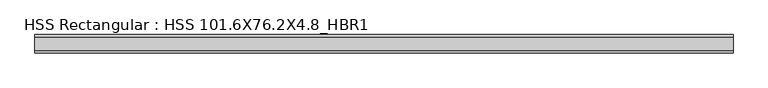
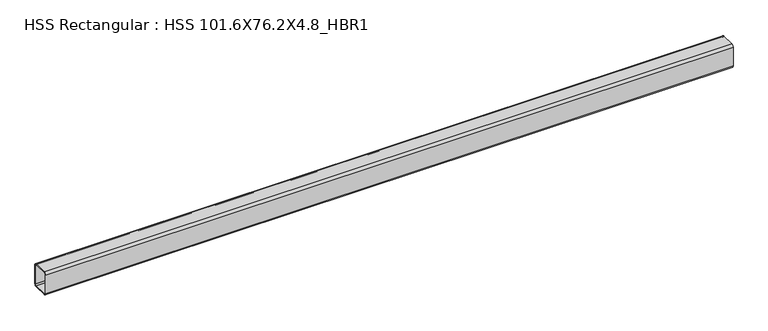
"""IFC4 building model written with IfcOpenShell, lengths in millimetres: beam geometry, HSS Rectangular : HSS 101.6X76.2X4.8_HBR1."""

from ifc_helpers import new_model, si_unit, point, frame, frame_2d, origin, place, context, project, spatial, polyline, circle_curve, trimmed, segment, composite_curve, outline, extrude, source, transform, mapped, element, save


def hss_rectangular_hss_101_6x76_2x4_8_hbr1_dbf90deb(model_context):
    return source(origin(), model_context, "Body", "SweptSolid", [
        extrude(outline(composite_curve([segment(polyline([(38.1, 41.275), (38.1, -41.275)]), True, "CONTINUOUS"), segment(trimmed(circle_curve(frame_2d((28.575, -41.275)), 9.525), [point((38.1, -41.275))], [point((28.575, -50.8))], False, "CARTESIAN"), True, "CONTINUOUS"), segment(polyline([(28.575, -50.8), (-28.575, -50.8)]), True, "CONTINUOUS"), segment(trimmed(circle_curve(frame_2d((-28.575, -41.275)), 9.525), [point((-28.575, -50.8))], [point((-38.1, -41.275))], False, "CARTESIAN"), True, "CONTINUOUS"), segment(polyline([(-38.1, -41.275), (-38.1, 41.275)]), True, "CONTINUOUS"), segment(trimmed(circle_curve(frame_2d((-28.575, 41.275)), 9.525), [point((-38.1, 41.275))], [point((-28.575, 50.8))], False, "CARTESIAN"), True, "CONTINUOUS"), segment(polyline([(-28.575, 50.8), (28.575, 50.8)]), True, "CONTINUOUS"), segment(trimmed(circle_curve(frame_2d((28.575, 41.275)), 9.525), [point((28.575, 50.8))], [point((38.1, 41.275))], False, "CARTESIAN"), True, "CONTINUOUS")], self_intersect=False), holes=[composite_curve([segment(trimmed(circle_curve(frame_2d((-28.575, 41.275)), 4.7625), [point((-28.575, 46.0375))], [point((-33.3375, 41.275))], True, "CARTESIAN"), True, "CONTINUOUS"), segment(polyline([(-33.3375, 41.275), (-33.3375, -41.275)]), True, "CONTINUOUS"), segment(trimmed(circle_curve(frame_2d((-28.575, -41.275)), 4.7625), [point((-33.3375, -41.275))], [point((-28.575, -46.0375))], True, "CARTESIAN"), True, "CONTINUOUS"), segment(polyline([(-28.575, -46.0375), (28.575, -46.0375)]), True, "CONTINUOUS"), segment(trimmed(circle_curve(frame_2d((28.575, -41.275)), 4.7625), [point((28.575, -46.0375))], [point((33.3375, -41.275))], True, "CARTESIAN"), True, "CONTINUOUS"), segment(polyline([(33.3375, -41.275), (33.3375, 41.275)]), True, "CONTINUOUS"), segment(trimmed(circle_curve(frame_2d((28.575, 41.275)), 4.7625), [point((33.3375, 41.275))], [point((28.575, 46.0375))], True, "CARTESIAN"), True, "CONTINUOUS"), segment(polyline([(28.575, 46.0375), (-28.575, 46.0375)]), True, "CONTINUOUS")], self_intersect=False)]), frame((-1376.6301953, 0.0, 0.0), z_axis=(1.0, 0.0, 0.0), x_axis=(0.0, 1.0, 0.0)), (0.0, 0.0, 1.0), 2906.597179),
    ])


if __name__ == "__main__":
    model = new_model("IFC4")
    model_context = context("Model", 3, world=origin())
    ifc_project = project(units=[si_unit("LENGTHUNIT", "METRE", prefix="MILLI")], contexts=[model_context])
    site = spatial("IfcSite", under=ifc_project)
    building = spatial("IfcBuilding", under=site)
    placement = place(None, origin())
    hss_rectangular_hss_101_6x76_2x4_8_hbr1_shape = hss_rectangular_hss_101_6x76_2x4_8_hbr1_dbf90deb(model_context)
    element("IfcBeam", 1, ObjectType="HSS Rectangular : HSS 101.6X76.2X4.8_HBR1", at=placement, inside=building, context=model_context, shape_type="MappedRepresentation", body=[
        mapped(hss_rectangular_hss_101_6x76_2x4_8_hbr1_shape, transform((0.0, 0.0, 0.0), x_axis=(1.0, 0.0, 0.0), y_axis=(0.0, 1.0, 0.0), z_axis=(0.0, 0.0, 1.0))),
    ])
    save(model, "model.ifc")

# Revit data of these elements
# Type "HSS Rectangular : HSS 101.6X76.2X4.8_HBR1"
#   Section Name Key = "HSS 4X3X3/16"
#   Assembly Code = "B10"
#   Width = 7.62 cm
#   Wall Nominal Thickness = 0.4763 cm
#   Wall Design Thickness = 0.442 cm
#   Torsional Moment of Inertia = 260.561 cm⁴
#   Torsional Modulus = 61.2876 cm³
#   Section Area = 14.4516 cm²
#   Plastic Modulus weak axis = 40.3122 cm³
#   Plastic Modulus strong axis = 49.1612 cm³
#   Perimeter = 0.881482 m²/m
#   Outer Fillet = 0.9525 cm
#   Nominal Weight = 12.1285 kgf/m
#   Moment of Inertia weak axis = 131.529 cm⁴
#   Moment of Inertia strong axis = 205.202 cm⁴
#   Inner Fillet = 0.4763 cm
#   Height = 10.16 cm
#   Elastic Modulus weak axis = 34.4128 cm³
#   Elastic Modulus strong axis = 40.476 cm³
#   Centroid Vertical = 5.08 cm
#   Centroid Horizontal = 3.81 cm
#   Length [instance default] = 1524 mm
#   Structural Material [instance default] = Steel ASTM A500, Grade B, Rectangular and Square
#   Principal Axes Angle = 0
# Element 1 (IfcBeam, "HSS Rectangular : HSS 101.6X76.2X4.8_HBR1")
#   Structural Material = Steel ASTM A992
#   Materials on its faces: "Steel ASTM A992"
# Materials
#   "Steel ASTM A500, Grade B, Rectangular and Square": class "Metal", colour RGB 199 199 199, transparency 0, Description = "Carbon steel", Cost = 0
#   "Steel ASTM A992": class "Metal", colour RGB 199 199 199, transparency 0, Description = "Structural steel 50ksi", Cost = 0
